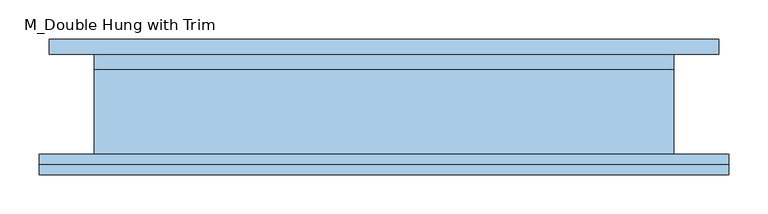
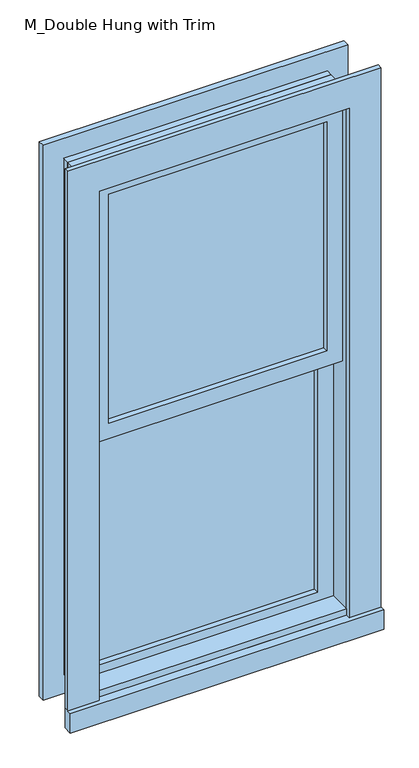
"""IFC4 building model written with IfcOpenShell, lengths in millimetres: window geometry, M_Double Hung with Trim."""

from ifc_helpers import new_model, si_unit, frame, origin, place, context, project, spatial, polyline, outline, extrude, source, transform, mapped, element, save


def m_double_hung_with_trim_fa2d897f(model_context):
    return source(origin(), model_context, "Body", "SweptSolid", [
        extrude(outline(polyline([(-304.8, 15.825), (-304.8, 28.525), (304.8, 28.525), (304.8, 15.825), (-304.8, 15.825)])), frame((0.0, 0.0, 628.65), z_axis=(0.0, 0.0, 1.0), x_axis=(1.0, 0.0, 0.0)), (0.0, 0.0, 1.0), 695.325),
        extrude(outline(polyline([(1368.425, -349.25), (584.2, -349.25), (584.2, 349.25), (1368.425, 349.25), (1368.425, -349.25)]), holes=[polyline([(1323.975, -304.8), (1323.975, 304.8), (628.65, 304.8), (628.65, -304.8), (1323.975, -304.8)])]), frame((0.0, -0.05, 0.0), z_axis=(0.0, 1.0, 0.0), x_axis=(0.0, 0.0, 1.0)), (0.0, 0.0, 1.0), 44.45),
        extrude(outline(polyline([(-438.25, -89.2), (-438.25, -63.5), (438.25, -63.5), (438.25, -89.2), (-438.25, -89.2)])), frame((0.0, 0.0, 526.95), z_axis=(0.0, 0.0, 1.0), x_axis=(1.0, 0.0, 0.0)), (0.0, 0.0, 1.0), 57.25),
        extrude(outline(polyline([(2178.15, -438.25), (526.95, -438.25), (526.95, 438.25), (2178.15, 438.25), (2178.15, -438.25)]), holes=[polyline([(2089.15, -349.25), (2089.15, 349.25), (584.2, 349.25), (584.2, -349.25), (2089.15, -349.25)])]), frame((0.0, -76.5, 0.0), z_axis=(0.0, 1.0, 0.0), x_axis=(0.0, 0.0, 1.0)), (0.0, 0.0, 1.0), 13.0),
        extrude(outline(polyline([(2165.45, 425.55), (2165.45, -425.55), (526.95, -425.55), (526.95, 425.55), (2165.45, 425.55)]), holes=[polyline([(2076.45, 336.55), (615.95, 336.55), (615.95, -336.55), (2076.45, -336.55), (2076.45, 336.55)])]), frame((0.0, 63.5, 0.0), z_axis=(0.0, 1.0, 0.0), x_axis=(0.0, 0.0, 1.0)), (0.0, 0.0, 1.0), 19.0),
        extrude(outline(polyline([(304.8, -15.925), (304.8, -28.625), (-304.8, -28.625), (-304.8, -15.925), (304.8, -15.925)])), frame((0.0, 0.0, 1368.425), z_axis=(0.0, 0.0, 1.0), x_axis=(1.0, 0.0, 0.0)), (0.0, 0.0, 1.0), 676.275),
        extrude(outline(polyline([(2089.15, -349.25), (1323.975, -349.25), (1323.975, 349.25), (2089.15, 349.25), (2089.15, -349.25)]), holes=[polyline([(2044.7, -304.8), (2044.7, 304.8), (1368.425, 304.8), (1368.425, -304.8), (2044.7, -304.8)])]), frame((0.0, -44.5, 0.0), z_axis=(0.0, 1.0, 0.0), x_axis=(0.0, 0.0, 1.0)), (0.0, 0.0, 1.0), 44.45),
        extrude(outline(polyline([(2108.2, -368.3), (584.2, -368.3), (584.2, 368.3), (2108.2, 368.3), (2108.2, -368.3)]), holes=[polyline([(2076.45, -336.55), (2076.45, 336.55), (615.95, 336.55), (615.95, -336.55), (2076.45, -336.55)])]), frame((0.0, 44.4, 0.0), z_axis=(0.0, 1.0, 0.0), x_axis=(0.0, 0.0, 1.0)), (0.0, 0.0, 1.0), 19.1),
        extrude(outline(polyline([(2108.2, 368.3), (2108.2, -368.3), (584.2, -368.3), (584.2, 368.3), (2108.2, 368.3)]), holes=[polyline([(2089.15, 349.25), (603.25, 349.25), (603.25, -349.25), (2089.15, -349.25), (2089.15, 349.25)])]), frame((0.0, -63.5, 0.0), z_axis=(0.0, 1.0, 0.0), x_axis=(0.0, 0.0, 1.0)), (0.0, 0.0, 1.0), 107.9),
    ])


if __name__ == "__main__":
    model = new_model("IFC4")
    model_context = context("Model", 3, world=origin())
    ifc_project = project(units=[si_unit("LENGTHUNIT", "METRE", prefix="MILLI")], contexts=[model_context])
    site = spatial("IfcSite", under=ifc_project)
    building = spatial("IfcBuilding", under=site)
    placement = place(None, origin())
    m_double_hung_with_trim_shape = m_double_hung_with_trim_fa2d897f(model_context)
    element("IfcWindow", 1, ObjectType="M_Double Hung with Trim : 29\" x 60\" @ 23\"", at=placement, inside=building, context=model_context, shape_type="MappedRepresentation", body=[
        mapped(m_double_hung_with_trim_shape, transform((0.0, 0.0, 0.0), x_axis=(1.0, 0.0, 0.0), y_axis=(0.0, 1.0, 0.0), z_axis=(0.0, 0.0, 1.0))),
    ])
    save(model, "model.ifc")

# Revit data of these elements
# Type "M_Double Hung with Trim : 29\" x 60\" @ 23\""
#   Type Mark = "61"
#   Construction Type Id = "GSP4R"
#   Analytic Construction = "1/8 in Pilkington single glazing"
#   Visual Light Transmittance = 0.9
#   Thermal Resistance (R) = 0.271106 (m²·K)/W
#   Solar Heat Gain Coefficient = 0.78
#   Heat Transfer Coefficient (U) = 3.6886 W/(m²·K)
#   Height = 5' - 0"
#   Default Sill Height = 1' - 11"
#   Trim Projection - Ext. = 0' - 0.51181"
#   Trim Projection - Int. = 0' - 0.74803"
#   Trim Width - Exterior = 0' - 3.50394"
#   Trim Width - Interior = 0' - 3.50394"
#   Width = 2' - 5"
#   Window Inset = 0' - 0.74803"
#   Glass Pane Material = EXISTING WINDOW
#   Sash = Trim
#   Trim Exterior Material = Trim
#   Trim Interior Material = Trim
#   Wall Closure = (empty or 0)
# Element 1 (IfcWindow, "M_Double Hung with Trim : 29\" x 60\" @ 23\"")
#   Materials on its faces: "Trim", "EXISTING WINDOW"
# Materials
#   "EXISTING WINDOW": class "Glass", colour RGB 218 227 224, transparency 0.85, Description = "Soda Lime Glass", Cost = 0
#   "Trim": class "Wood", colour RGB 250 251 245, transparency 0, Cost = 0
